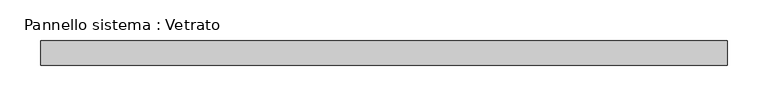
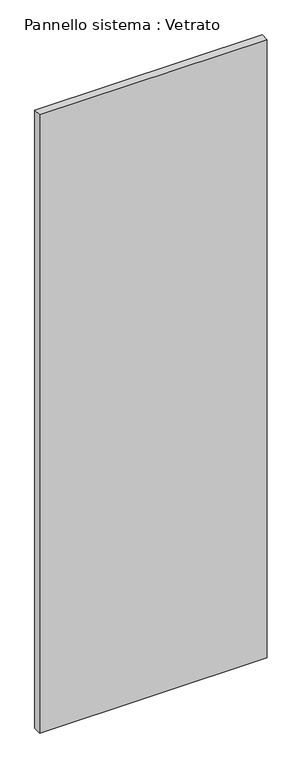
"""IFC4 building model written with IfcOpenShell, lengths in millimetres: plate geometry, Pannello sistema : Vetrato."""

from ifc_helpers import new_model, si_unit, origin, origin_with_axes, place, context, project, spatial, polyline, outline, extrude, source, transform, mapped, element, save


def pannello_sistema_vetrato_33ed3eaa(model_context):
    return source(origin(), model_context, "Body", "SweptSolid", [
        extrude(outline(polyline([(422.5, -15.0), (-422.5, -15.0), (-422.5, 15.0), (422.5, 15.0), (422.5, -15.0)])), origin_with_axes(), (0.0, 0.0, 1.0), 2425.0),
    ])


if __name__ == "__main__":
    model = new_model("IFC4")
    model_context = context("Model", 3, world=origin())
    ifc_project = project(units=[si_unit("LENGTHUNIT", "METRE", prefix="MILLI")], contexts=[model_context])
    site = spatial("IfcSite", under=ifc_project)
    building = spatial("IfcBuilding", under=site)
    placement = place(None, origin())
    pannello_sistema_vetrato_shape = pannello_sistema_vetrato_33ed3eaa(model_context)
    element("IfcPlate", 1, ObjectType="Pannello sistema : Vetrato", at=placement, inside=building, context=model_context, shape_type="MappedRepresentation", body=[
        mapped(pannello_sistema_vetrato_shape, transform((0.0, 0.0, 0.0), x_axis=(1.0, 0.0, 0.0), y_axis=(0.0, 1.0, 0.0), z_axis=(0.0, 0.0, 1.0))),
    ])
    save(model, "model.ifc")

# Revit data of these elements
# Type "Pannello sistema : Vetrato"
#   Construction Type Id = "GSP4R"
#   Analytic Construction = "Vetrata singola Pilkington 1/8 in"
#   Visual Light Transmittance = 0.9
#   Solar Heat Gain Coefficient = 0.86
#   Heat Transfer Coefficient (U) = 6.7069 W/(m²·K)
# Element 1 (IfcPlate, "Pannello sistema : Vetrato")
#   Materials on its faces: "Default - Vetro"
# Materials
#   "Default - Vetro": class "Vetro", colour RGB 208 208 208, transparency 0.7, Cost = 0
